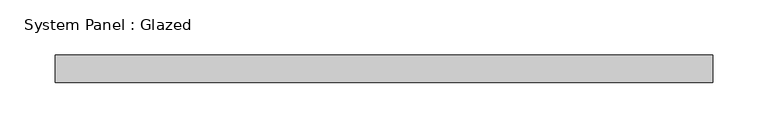
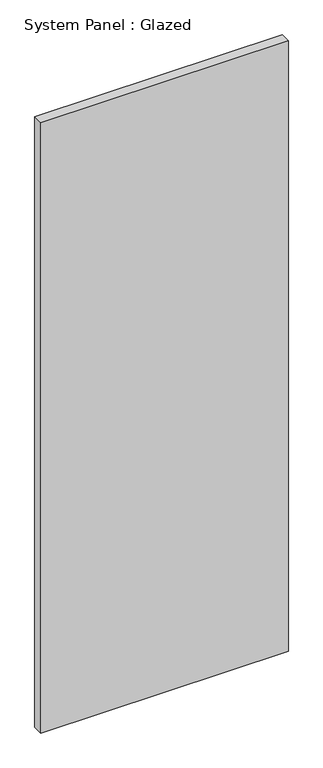
"""IFC4 building model written with IfcOpenShell, lengths in millimetres: plate geometry, System Panel : Glazed."""

from ifc_helpers import new_model, si_unit, origin, origin_with_axes, place, context, project, spatial, polyline, outline, extrude, source, transform, mapped, element, save


def system_panel_glazed_85002481(model_context):
    return source(origin(), model_context, "Body", "SweptSolid", [
        extrude(outline(polyline([(297.5, 24.5), (-297.5, 24.5), (-297.5, 49.5), (297.5, 49.5), (297.5, 24.5)])), origin_with_axes(), (0.0, 0.0, 1.0), 1550.0),
    ])


if __name__ == "__main__":
    model = new_model("IFC4")
    model_context = context("Model", 3, world=origin())
    ifc_project = project(units=[si_unit("LENGTHUNIT", "METRE", prefix="MILLI")], contexts=[model_context])
    site = spatial("IfcSite", under=ifc_project)
    building = spatial("IfcBuilding", under=site)
    placement = place(None, origin())
    system_panel_glazed_shape = system_panel_glazed_85002481(model_context)
    element("IfcPlate", 1, ObjectType="System Panel : Glazed", at=placement, inside=building, context=model_context, shape_type="MappedRepresentation", body=[
        mapped(system_panel_glazed_shape, transform((0.0, 0.0, 0.0), x_axis=(1.0, 0.0, 0.0), y_axis=(0.0, 1.0, 0.0), z_axis=(0.0, 0.0, 1.0))),
    ])
    save(model, "model.ifc")

# Revit data of these elements
# Element 1 (IfcPlate, "System Panel : Glazed")
#   Materials on its faces: "Glass"
# Materials
#   "Glass": class "Glass", colour RGB 0 128 192, transparency 0.9
